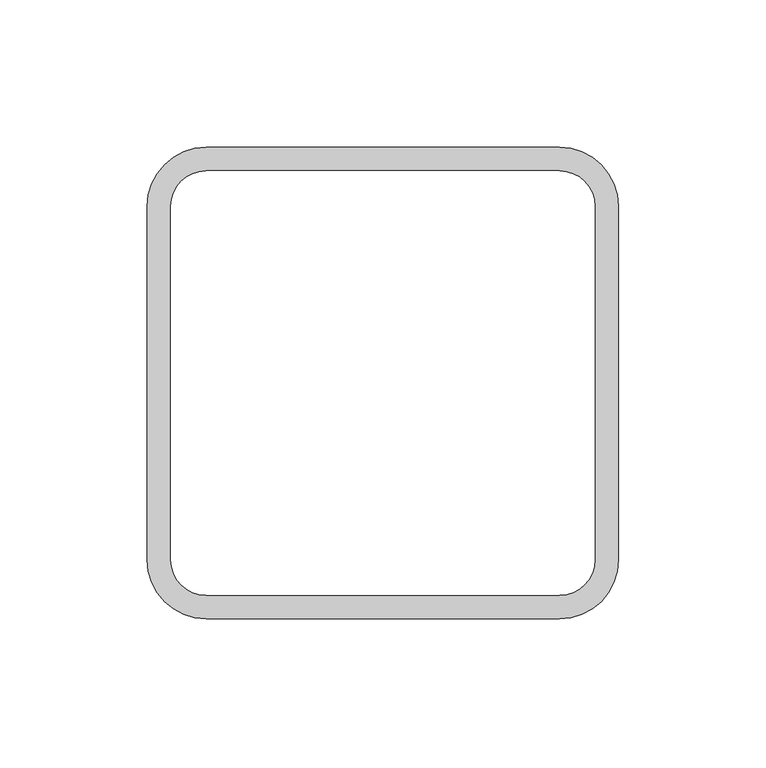
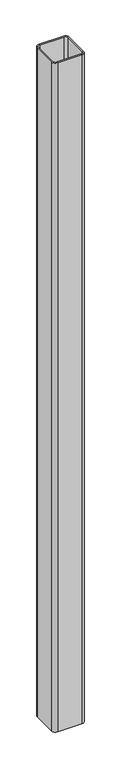
"""IFC4 building model written with IfcOpenShell, lengths in millimetres: column geometry, NLRS_28_SCO_TLB_stalen kolom buisprofiel koudgevormd vierkant-BCPG-MMBS-SRP_gen_rsf : stalen kolom buisprofiel koudgevormd vierkant RHSC_gen__160x160x8."""

from ifc_helpers import new_model, si_unit, point, frame, frame_2d, origin, place, context, project, spatial, polyline, circle_curve, trimmed, segment, composite_curve, outline, extrude, source, transform, mapped, element, save


def column_9b451431(model_context):
    return source(origin(), model_context, "Body", "SweptSolid", [
        extrude(outline(composite_curve([segment(trimmed(circle_curve(frame_2d((60.0, 60.0)), 20.0), [point((60.0, 80.0))], [point((80.0, 60.0))], False, "CARTESIAN"), True, "CONTINUOUS"), segment(polyline([(80.0, 60.0), (80.0, -60.0)]), True, "CONTINUOUS"), segment(trimmed(circle_curve(frame_2d((60.0, -60.0)), 20.0), [point((80.0, -60.0))], [point((60.0, -80.0))], False, "CARTESIAN"), True, "CONTINUOUS"), segment(polyline([(60.0, -80.0), (-60.0, -80.0)]), True, "CONTINUOUS"), segment(trimmed(circle_curve(frame_2d((-60.0, -60.0)), 20.0), [point((-60.0, -80.0))], [point((-80.0, -60.0))], False, "CARTESIAN"), True, "CONTINUOUS"), segment(polyline([(-80.0, -60.0), (-80.0, 60.0)]), True, "CONTINUOUS"), segment(trimmed(circle_curve(frame_2d((-60.0, 60.0)), 20.0), [point((-80.0, 60.0))], [point((-60.0, 80.0))], False, "CARTESIAN"), True, "CONTINUOUS"), segment(polyline([(-60.0, 80.0), (60.0, 80.0)]), True, "CONTINUOUS")], self_intersect=False), holes=[composite_curve([segment(polyline([(60.0, 72.0), (-60.0, 72.0)]), True, "CONTINUOUS"), segment(trimmed(circle_curve(frame_2d((-60.0, 60.0)), 12.0), [point((-60.0, 72.0))], [point((-72.0, 60.0))], True, "CARTESIAN"), True, "CONTINUOUS"), segment(polyline([(-72.0, 60.0), (-72.0, -60.0)]), True, "CONTINUOUS"), segment(trimmed(circle_curve(frame_2d((-60.0, -60.0)), 12.0), [point((-72.0, -60.0))], [point((-60.0, -72.0))], True, "CARTESIAN"), True, "CONTINUOUS"), segment(polyline([(-60.0, -72.0), (60.0, -72.0)]), True, "CONTINUOUS"), segment(trimmed(circle_curve(frame_2d((60.0, -60.0)), 12.0), [point((60.0, -72.0))], [point((72.0, -60.0))], True, "CARTESIAN"), True, "CONTINUOUS"), segment(polyline([(72.0, -60.0), (72.0, 60.0)]), True, "CONTINUOUS"), segment(trimmed(circle_curve(frame_2d((60.0, 60.0)), 12.0), [point((72.0, 60.0))], [point((60.0, 72.0))], True, "CARTESIAN"), True, "CONTINUOUS")], self_intersect=False)]), frame((0.0, 0.0, 7560.0), z_axis=(0.0, 0.0, 1.0), x_axis=(1.0, 0.0, 0.0)), (0.0, 0.0, 1.0), 3510.0),
    ])


if __name__ == "__main__":
    model = new_model("IFC4")
    model_context = context("Model", 3, world=origin())
    ifc_project = project(units=[si_unit("LENGTHUNIT", "METRE", prefix="MILLI")], contexts=[model_context])
    site = spatial("IfcSite", under=ifc_project)
    building = spatial("IfcBuilding", under=site)
    placement = place(None, origin())
    column_shape = column_9b451431(model_context)
    element("IfcColumn", 1, ObjectType="NLRS_28_SCO_TLB_stalen kolom buisprofiel koudgevormd vierkant-BCPG-MMBS-SRP_gen_rsf : stalen kolom buisprofiel koudgevormd vierkant RHSC_gen__160x160x8", at=placement, inside=building, context=model_context, shape_type="MappedRepresentation", body=[
        mapped(column_shape, transform((0.0, 0.0, 0.0), x_axis=(1.0, 0.0, 0.0), y_axis=(0.0, 1.0, 0.0), z_axis=(0.0, 0.0, 1.0))),
    ])
    save(model, "model.ifc")

# Revit data of these elements
# Type "NLRS_28_SCO_TLB_stalen kolom buisprofiel koudgevormd vierkant-BCPG-MMBS-SRP_gen_rsf : stalen kolom buisprofiel koudgevormd vierkant RHSC_gen__160x160x8"
#   Type IfcGUID = "2$hNzCXOT3YR8V$0Cfyzxk"
#   IfcExportAs = "IfcColumnType"
#   IfcExportType = "COLUMN"
#   Type Comments = "K160x160x8"
#   Model = " "
#   Manufacturer = " "
#   Description = "stalen kolom K160x160x8"
#   Assembly Code = "28.11"
#   vz = 80 mm
#   vy = 80 mm
#   vpz = 80 mm
#   vpy = 80 mm
#   tw = 8 mm
#   tf = 8 mm
#   ri = 20 mm
#   ra = 12 mm
#   d = 160 mm
#   bf = 160 mm
#   NLRS_C_lengte [instance default] = 2743.2 mm
#   Structural Material = NLRS_h2_staal_gen_rsf
#   Keynote = ""
# Element 1 (IfcColumn, "NLRS_28_SCO_TLB_stalen kolom buisprofiel koudgevormd vierkant-BCPG-MMBS-SRP_gen_rsf : stalen kolom buisprofiel koudgevormd vierkant RHSC_gen__160x160x8")
#   NLRS_C_lengte = 3510 mm
#   Materials on its faces: "NLRS_h2_staal_gen_rsf"
# Materials
#   "NLRS_h2_staal_gen_rsf": class "H - Metaal", colour RGB 189 187 185, transparency 0, Keynote = "h2", Manufacturer = "Revit Standards Foundation", URL = "www.revitstandards.org", Description = "staal", Cost = 0
